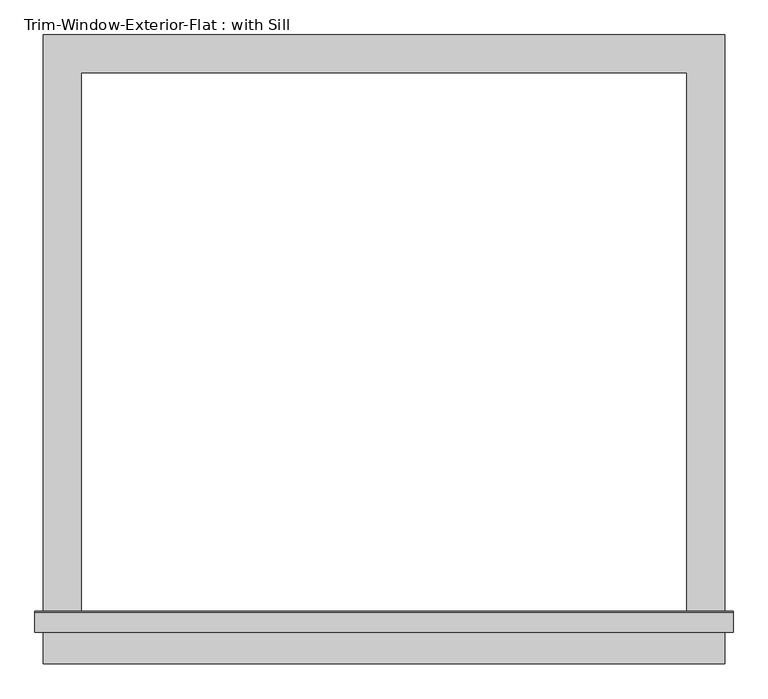
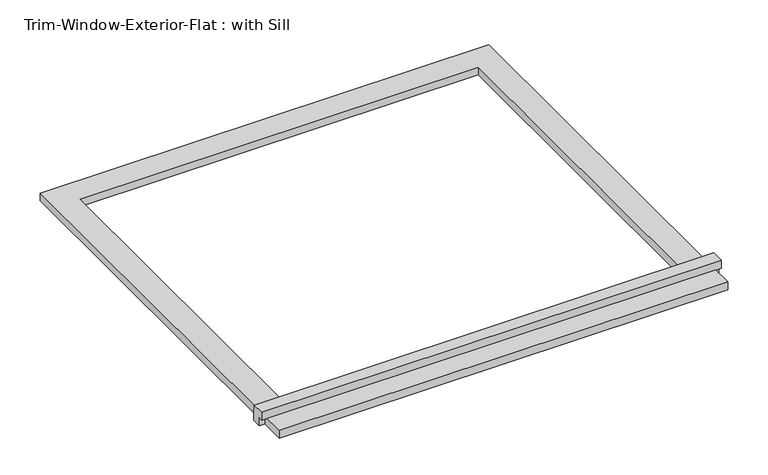
"""IFC4 building model written with IfcOpenShell, lengths in millimetres: proxy geometry, Trim-Window-Exterior-Flat : with Sill."""

from ifc_helpers import new_model, si_unit, frame, origin, origin_with_axes, place, context, project, spatial, polyline, outline, extrude, source, transform, mapped, element, save


def trim_window_exterior_flat_with_sill_49d6f9d6(model_context):
    return source(origin(), model_context, "Body", "SweptSolid", [
        extrude(outline(polyline([(514.35, -834.9823709), (514.35, -892.1323709), (-514.35, -892.1323709), (-514.35, -834.9823709), (514.35, -834.9823709)])), origin_with_axes(), (0.0, 0.0, 1.0), 19.05),
        extrude(outline(polyline([(-844.55, 38.1), (-815.2580645, 38.1), (-812.8, 19.05), (-812.8, 0.0), (-834.9823709, 0.0), (-834.9823709, 19.05), (-844.55, 19.05), (-844.55, 38.1)])), frame((-527.05, 0.0, 0.0), z_axis=(1.0, 0.0, 0.0), x_axis=(0.0, 1.0, 0.0)), (0.0, 0.0, 1.0), 1054.1),
        extrude(outline(polyline([(-514.35, 57.15), (514.35, 57.15), (514.35, -812.8), (457.2, -812.8), (457.2, 0.0), (-457.2, 0.0), (-457.2, -812.8), (-514.35, -812.8), (-514.35, 57.15)])), origin_with_axes(), (0.0, 0.0, 1.0), 19.05),
    ])


if __name__ == "__main__":
    model = new_model("IFC4")
    model_context = context("Model", 3, world=origin())
    ifc_project = project(units=[si_unit("LENGTHUNIT", "METRE", prefix="MILLI")], contexts=[model_context])
    site = spatial("IfcSite", under=ifc_project)
    building = spatial("IfcBuilding", under=site)
    placement = place(None, origin())
    trim_window_exterior_flat_with_sill_shape = trim_window_exterior_flat_with_sill_49d6f9d6(model_context)
    element("IfcBuildingElementProxy", 1, Name="Trim-Window-Exterior-Flat : with Sill", ObjectType="Trim-Window-Exterior-Flat : with Sill", at=placement, inside=building, context=model_context, shape_type="MappedRepresentation", body=[
        mapped(trim_window_exterior_flat_with_sill_shape, transform((0.0, 0.0, 0.0), x_axis=(1.0, 0.0, 0.0), y_axis=(0.0, 1.0, 0.0), z_axis=(0.0, 0.0, 1.0))),
    ])
    save(model, "model.ifc")

# Revit data of these elements
# Type "Trim-Window-Exterior-Flat : with Sill"
#   Trim Width = 0' - 2 1/4"
#   Trim Thickness_Picture Frame = 0' - 1 1/4"
#   Trim Thickness_with Sill = 0' - 0 3/4"
#   Sill Thickness = 0' - 1 1/4"
#   Opening Width [instance default] = 2' - 0"
#   Opening Height [instance default] = 3' - 0"
#   Default Elevation = 4' - 0"
#   Sill = yes
#   Picture Frame = no
#   Trim Material [instance default] = none
# Element 1 (IfcBuildingElementProxy, "Trim-Window-Exterior-Flat : with Sill")
#   Opening Width = 3' - 0"
#   Opening Height = 2' - 8"
#   Trim Material = Clad - White
#   Materials on its faces: "Clad - White"
# Materials
#   "Clad - White": class "Wood", colour RGB 245 245 243, transparency 0, Cost = 0
